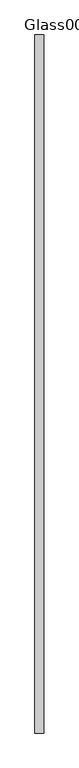
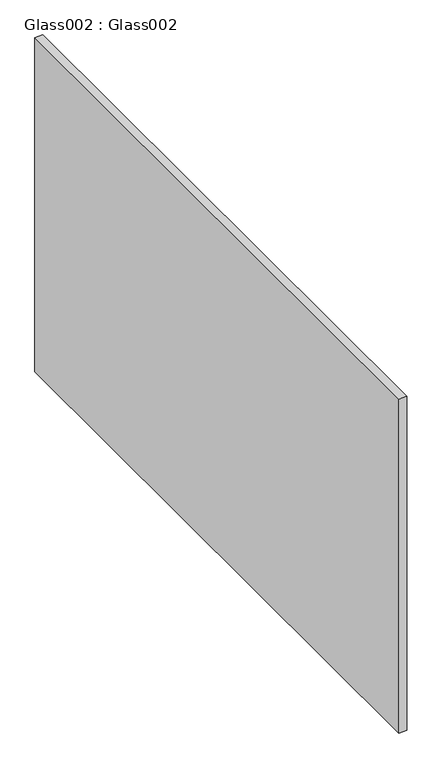
"""IFC4 building model written with IfcOpenShell, lengths in millimetres: proxy geometry, Glass002 : Glass002."""

from ifc_helpers import new_model, si_unit, frame, origin, place, context, project, spatial, polyline, outline, extrude, source, transform, mapped, element, save


def glass002_glass002_cd7bb274(model_context):
    return source(origin(), model_context, "Body", "SweptSolid", [
        extrude(outline(polyline([(-7059.8834918, 7982.1531721), (-7085.0334918, 7982.1531721), (-7085.0334918, 9982.1531721), (-7059.8834918, 9982.1531721), (-7059.8834918, 7982.1531721)])), frame((0.0, 0.0, 40149.5092895), z_axis=(0.0, 0.0, 1.0), x_axis=(1.0, 0.0, 0.0)), (0.0, 0.0, 1.0), 1120.65),
    ])


if __name__ == "__main__":
    model = new_model("IFC4")
    model_context = context("Model", 3, world=origin())
    ifc_project = project(units=[si_unit("LENGTHUNIT", "METRE", prefix="MILLI")], contexts=[model_context])
    site = spatial("IfcSite", under=ifc_project)
    building = spatial("IfcBuilding", under=site)
    placement = place(None, origin())
    glass002_glass002_shape = glass002_glass002_cd7bb274(model_context)
    element("IfcBuildingElementProxy", 1, Name="Glass002 : Glass002", ObjectType="Glass002 : Glass002", at=placement, inside=building, context=model_context, shape_type="MappedRepresentation", body=[
        mapped(glass002_glass002_shape, transform((0.0, 0.0, 0.0), x_axis=(1.0, 0.0, 0.0), y_axis=(0.0, 1.0, 0.0), z_axis=(0.0, 0.0, 1.0))),
    ])
    save(model, "model.ifc")

# Revit data of these elements
# Type "Glass002 : Glass002"
#   NameOverride = "Glass002"
# Element 1 (IfcBuildingElementProxy, "Glass002 : Glass002")
#   Materials on its faces: "GLASS RAILING TBD"
# Materials
#   "GLASS RAILING TBD": class "Unassigned", colour RGB 64 209 242, transparency 0
